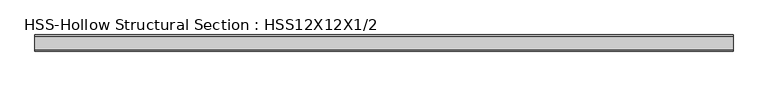
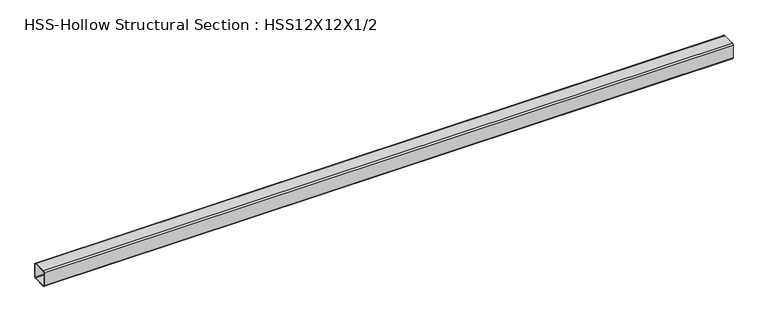
"""IFC4 building model written with IfcOpenShell, lengths in millimetres: beam geometry, HSS-Hollow Structural Section : HSS12X12X1/2."""

from ifc_helpers import new_model, si_unit, point, frame, frame_2d, origin, place, context, project, spatial, polyline, circle_curve, trimmed, segment, composite_curve, outline, extrude, source, transform, mapped, element, save


def hss_hollow_structural_section_hss12x12x1_2_65790d26(model_context):
    return source(origin(), model_context, "Body", "SweptSolid", [
        extrude(outline(composite_curve([segment(polyline([(152.4, 128.778), (152.4, -128.778)]), True, "CONTINUOUS"), segment(trimmed(circle_curve(frame_2d((128.778, -128.778)), 23.622), [point((152.4, -128.778))], [point((128.778, -152.4))], False, "CARTESIAN"), True, "CONTINUOUS"), segment(polyline([(128.778, -152.4), (-128.778, -152.4)]), True, "CONTINUOUS"), segment(trimmed(circle_curve(frame_2d((-128.778, -128.778)), 23.622), [point((-128.778, -152.4))], [point((-152.4, -128.778))], False, "CARTESIAN"), True, "CONTINUOUS"), segment(polyline([(-152.4, -128.778), (-152.4, 128.778)]), True, "CONTINUOUS"), segment(trimmed(circle_curve(frame_2d((-128.778, 128.778)), 23.622), [point((-152.4, 128.778))], [point((-128.778, 152.4))], False, "CARTESIAN"), True, "CONTINUOUS"), segment(polyline([(-128.778, 152.4), (128.778, 152.4)]), True, "CONTINUOUS"), segment(trimmed(circle_curve(frame_2d((128.778, 128.778)), 23.622), [point((128.778, 152.4))], [point((152.4, 128.778))], False, "CARTESIAN"), True, "CONTINUOUS")], self_intersect=False), holes=[composite_curve([segment(trimmed(circle_curve(frame_2d((-128.778, 128.778)), 11.811), [point((-128.778, 140.589))], [point((-140.589, 128.778))], True, "CARTESIAN"), True, "CONTINUOUS"), segment(polyline([(-140.589, 128.778), (-140.589, -128.778)]), True, "CONTINUOUS"), segment(trimmed(circle_curve(frame_2d((-128.778, -128.778)), 11.811), [point((-140.589, -128.778))], [point((-128.778, -140.589))], True, "CARTESIAN"), True, "CONTINUOUS"), segment(polyline([(-128.778, -140.589), (128.778, -140.589)]), True, "CONTINUOUS"), segment(trimmed(circle_curve(frame_2d((128.778, -128.778)), 11.811), [point((128.778, -140.589))], [point((140.589, -128.778))], True, "CARTESIAN"), True, "CONTINUOUS"), segment(polyline([(140.589, -128.778), (140.589, 128.778)]), True, "CONTINUOUS"), segment(trimmed(circle_curve(frame_2d((128.778, 128.778)), 11.811), [point((140.589, 128.778))], [point((128.778, 140.589))], True, "CARTESIAN"), True, "CONTINUOUS"), segment(polyline([(128.778, 140.589), (-128.778, 140.589)]), True, "CONTINUOUS")], self_intersect=False)]), frame((-6674.2846052, 0.0, 0.0), z_axis=(1.0, 0.0, 0.0), x_axis=(0.0, 1.0, 0.0)), (0.0, 0.0, 1.0), 13185.2516926),
    ])


if __name__ == "__main__":
    model = new_model("IFC4")
    model_context = context("Model", 3, world=origin())
    ifc_project = project(units=[si_unit("LENGTHUNIT", "METRE", prefix="MILLI")], contexts=[model_context])
    site = spatial("IfcSite", under=ifc_project)
    building = spatial("IfcBuilding", under=site)
    placement = place(None, origin())
    hss_hollow_structural_section_hss12x12x1_2_shape = hss_hollow_structural_section_hss12x12x1_2_65790d26(model_context)
    element("IfcBeam", 1, ObjectType="HSS-Hollow Structural Section : HSS12X12X1/2", at=placement, inside=building, context=model_context, shape_type="MappedRepresentation", body=[
        mapped(hss_hollow_structural_section_hss12x12x1_2_shape, transform((0.0, 0.0, 0.0), x_axis=(1.0, 0.0, 0.0), y_axis=(0.0, 1.0, 0.0), z_axis=(0.0, 0.0, 1.0))),
    ])
    save(model, "model.ifc")

# Revit data of these elements
# Type "HSS-Hollow Structural Section : HSS12X12X1/2"
#   Assembly Code = "B10"
#   Shape = "Square"
#   W = 75.9
#   Ht = 304.8 mm
#   Length [instance default] = 1524 mm
#   b = 304.8 mm
#   kr = 23.622 mm
#   t = 11.811 mm
#   A = 0.0134838 m²
#   Structural Material [instance default] = Steel ASTM A500, Grade B, Rectangular and Square
# Element 1 (IfcBeam, "HSS-Hollow Structural Section : HSS12X12X1/2")
#   Structural Material = Aluminum 7175 T73 0 Hot Formed
#   Materials on its faces: "Aluminum 7175 T73 0 Hot Formed"
# Materials
#   "Steel ASTM A500, Grade B, Rectangular and Square": class "Metal", colour RGB 199 199 199, transparency 0, Description = "Carbon steel", Cost = 0
#   "Aluminum 7175 T73 0 Hot Formed": class "Metal", colour RGB 120 120 120, transparency 0, Description = "Physical material.", Cost = 0
